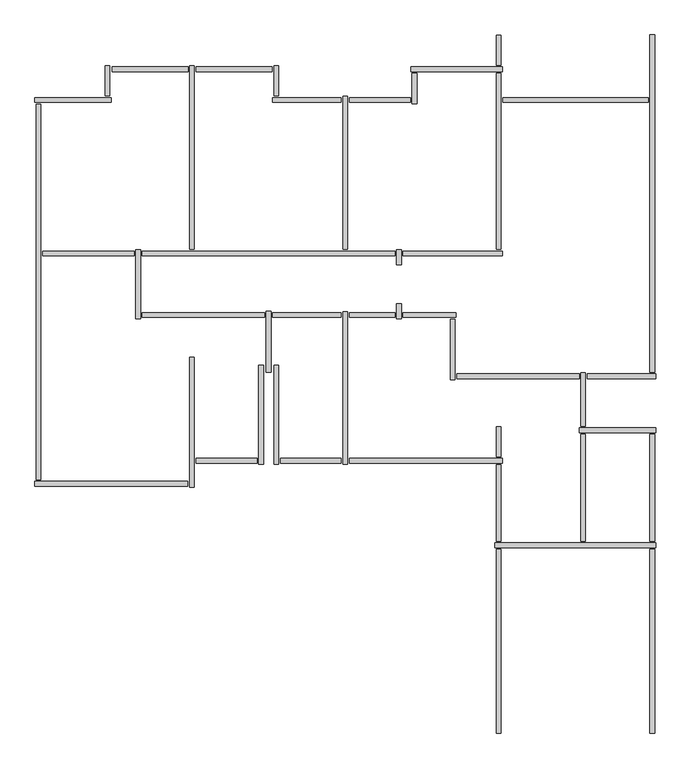
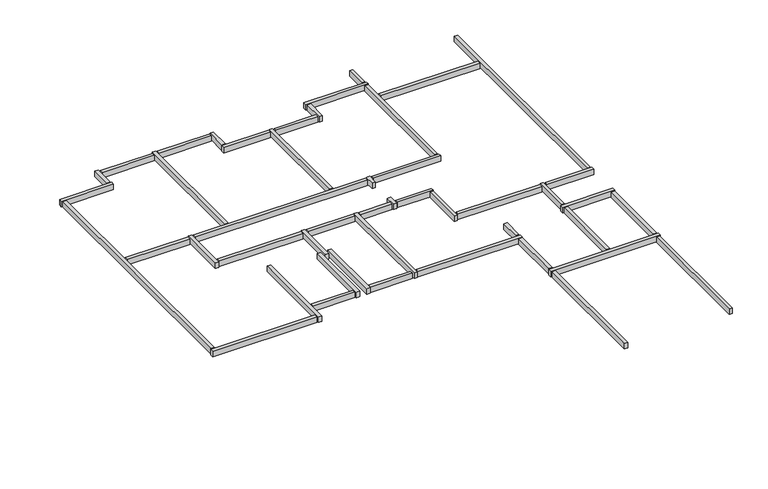
"""IFC4 building model written with IfcOpenShell, lengths in millimetres: beam geometry, Graute viga de respaldo19 : Graute viga de respaldo."""

from ifc_helpers import new_model, si_unit, frame, origin, place, context, project, spatial, polyline, outline, extrude, source, transform, mapped, element, save


def beam_b2c9fdfa(model_context):
    return source(origin(), model_context, "Body", "SweptSolid", [
        extrude(outline(polyline([(-70718.7587292, 62785.4278788), (-70624.7587292, 62785.4278788), (-70624.7587292, 59195.4278788), (-70718.7587292, 59195.4278788), (-70718.7587292, 62785.4278788)])), frame((0.0, 0.0, 14632.9999999), z_axis=(0.0, 0.0, 1.0), x_axis=(1.0, 0.0, 0.0)), (0.0, 0.0, 1.0), 167.0),
        extrude(outline(polyline([(-67718.7587292, 62785.4278788), (-67624.7587292, 62785.4278788), (-67624.7587292, 59195.4278788), (-67718.7587292, 59195.4278788), (-67718.7587292, 62785.4278788)])), frame((0.0, 0.0, 14632.9999999), z_axis=(0.0, 0.0, 1.0), x_axis=(1.0, 0.0, 0.0)), (0.0, 0.0, 1.0), 167.0),
        extrude(outline(polyline([(-75401.7587292, 64562.4278788), (-75401.7587292, 64468.4278788), (-76591.7587292, 64468.4278788), (-76591.7587292, 64562.4278788), (-75401.7587292, 64562.4278788)])), frame((0.0, 0.0, 14632.9999999), z_axis=(0.0, 0.0, 1.0), x_axis=(1.0, 0.0, 0.0)), (0.0, 0.0, 1.0), 167.0),
        extrude(outline(polyline([(-73751.7587292, 64562.4278788), (-73751.7587292, 64468.4278788), (-74941.7587292, 64468.4278788), (-74941.7587292, 64562.4278788), (-73751.7587292, 64562.4278788)])), frame((0.0, 0.0, 14632.9999999), z_axis=(0.0, 0.0, 1.0), x_axis=(1.0, 0.0, 0.0)), (0.0, 0.0, 1.0), 167.0),
        extrude(outline(polyline([(-77801.7587292, 68612.4278788), (-77801.7587292, 68518.4278788), (-79591.7587292, 68518.4278788), (-79591.7587292, 68612.4278788), (-77801.7587292, 68612.4278788)])), frame((0.0, 0.0, 14632.9999999), z_axis=(0.0, 0.0, 1.0), x_axis=(1.0, 0.0, 0.0)), (0.0, 0.0, 1.0), 167.0),
        extrude(outline(polyline([(-72401.7587292, 71612.4278788), (-72401.7587292, 71518.4278788), (-73591.7587292, 71518.4278788), (-73591.7587292, 71612.4278788), (-72401.7587292, 71612.4278788)])), frame((0.0, 0.0, 14632.9999999), z_axis=(0.0, 0.0, 1.0), x_axis=(1.0, 0.0, 0.0)), (0.0, 0.0, 1.0), 167.0),
        extrude(outline(polyline([(-72274.7587292, 71495.4278788), (-72368.7587292, 71495.4278788), (-72368.7587292, 72085.4278788), (-72274.7587292, 72085.4278788), (-72274.7587292, 71495.4278788)])), frame((0.0, 0.0, 14632.9999999), z_axis=(0.0, 0.0, 1.0), x_axis=(1.0, 0.0, 0.0)), (0.0, 0.0, 1.0), 167.0),
        extrude(outline(polyline([(-70601.7587292, 72212.4278788), (-70601.7587292, 72118.4278788), (-72391.7587292, 72118.4278788), (-72391.7587292, 72212.4278788), (-70601.7587292, 72212.4278788)])), frame((0.0, 0.0, 14632.9999999), z_axis=(0.0, 0.0, 1.0), x_axis=(1.0, 0.0, 0.0)), (0.0, 0.0, 1.0), 167.0),
        extrude(outline(polyline([(-72668.7587292, 68635.4278788), (-72574.7587292, 68635.4278788), (-72574.7587292, 68345.4278788), (-72668.7587292, 68345.4278788), (-72668.7587292, 68635.4278788)])), frame((0.0, 0.0, 14632.9999999), z_axis=(0.0, 0.0, 1.0), x_axis=(1.0, 0.0, 0.0)), (0.0, 0.0, 1.0), 167.0),
        extrude(outline(polyline([(-75251.7587292, 67412.4278788), (-75251.7587292, 67318.4278788), (-77641.7587292, 67318.4278788), (-77641.7587292, 67412.4278788), (-75251.7587292, 67412.4278788)])), frame((0.0, 0.0, 14632.9999999), z_axis=(0.0, 0.0, 1.0), x_axis=(1.0, 0.0, 0.0)), (0.0, 0.0, 1.0), 167.0),
        extrude(outline(polyline([(-73751.7587292, 67412.4278788), (-73751.7587292, 67318.4278788), (-75091.7587292, 67318.4278788), (-75091.7587292, 67412.4278788), (-73751.7587292, 67412.4278788)])), frame((0.0, 0.0, 14632.9999999), z_axis=(0.0, 0.0, 1.0), x_axis=(1.0, 0.0, 0.0)), (0.0, 0.0, 1.0), 167.0),
        extrude(outline(polyline([(-72701.7587292, 67412.4278788), (-72701.7587292, 67318.4278788), (-73591.7587292, 67318.4278788), (-73591.7587292, 67412.4278788), (-72701.7587292, 67412.4278788)])), frame((0.0, 0.0, 14632.9999999), z_axis=(0.0, 0.0, 1.0), x_axis=(1.0, 0.0, 0.0)), (0.0, 0.0, 1.0), 167.0),
        extrude(outline(polyline([(-72668.7587292, 67585.4278788), (-72574.7587292, 67585.4278788), (-72574.7587292, 67295.4278788), (-72668.7587292, 67295.4278788), (-72668.7587292, 67585.4278788)])), frame((0.0, 0.0, 14632.9999999), z_axis=(0.0, 0.0, 1.0), x_axis=(1.0, 0.0, 0.0)), (0.0, 0.0, 1.0), 167.0),
        extrude(outline(polyline([(-71511.7587292, 67412.4278788), (-71511.7587292, 67318.4278788), (-72541.7587292, 67318.4278788), (-72541.7587292, 67412.4278788), (-71511.7587292, 67412.4278788)])), frame((0.0, 0.0, 14632.9999999), z_axis=(0.0, 0.0, 1.0), x_axis=(1.0, 0.0, 0.0)), (0.0, 0.0, 1.0), 167.0),
        extrude(outline(polyline([(-71524.7587292, 66095.4278788), (-71618.7587292, 66095.4278788), (-71618.7587292, 67285.4278788), (-71524.7587292, 67285.4278788), (-71524.7587292, 66095.4278788)])), frame((0.0, 0.0, 14632.9999999), z_axis=(0.0, 0.0, 1.0), x_axis=(1.0, 0.0, 0.0)), (0.0, 0.0, 1.0), 167.0),
        extrude(outline(polyline([(-69091.7587292, 66212.4278788), (-69091.7587292, 66118.4278788), (-71491.7587292, 66118.4278788), (-71491.7587292, 66212.4278788), (-69091.7587292, 66212.4278788)])), frame((0.0, 0.0, 14632.9999999), z_axis=(0.0, 0.0, 1.0), x_axis=(1.0, 0.0, 0.0)), (0.0, 0.0, 1.0), 167.0),
        extrude(outline(polyline([(-73718.7587292, 67430.4278788), (-73624.7587292, 67430.4278788), (-73624.7587292, 64445.4278788), (-73718.7587292, 64445.4278788), (-73718.7587292, 67430.4278788)])), frame((0.0, 0.0, 14632.9999999), z_axis=(0.0, 0.0, 1.0), x_axis=(1.0, 0.0, 0.0)), (0.0, 0.0, 1.0), 167.0),
        extrude(outline(polyline([(-70601.7587292, 64562.4278788), (-70601.7587292, 64468.4278788), (-73591.7587292, 64468.4278788), (-73591.7587292, 64562.4278788), (-70601.7587292, 64562.4278788)])), frame((0.0, 0.0, 14632.9999999), z_axis=(0.0, 0.0, 1.0), x_axis=(1.0, 0.0, 0.0)), (0.0, 0.0, 1.0), 167.0),
        extrude(outline(polyline([(-70718.7587292, 65185.4278788), (-70624.7587292, 65185.4278788), (-70624.7587292, 64595.4278788), (-70718.7587292, 64595.4278788), (-70718.7587292, 65185.4278788)])), frame((0.0, 0.0, 14632.9999999), z_axis=(0.0, 0.0, 1.0), x_axis=(1.0, 0.0, 0.0)), (0.0, 0.0, 1.0), 167.0),
        extrude(outline(polyline([(-70624.7587292, 62945.4278788), (-70718.7587292, 62945.4278788), (-70718.7587292, 64435.4278788), (-70624.7587292, 64435.4278788), (-70624.7587292, 62945.4278788)])), frame((0.0, 0.0, 14632.9999999), z_axis=(0.0, 0.0, 1.0), x_axis=(1.0, 0.0, 0.0)), (0.0, 0.0, 1.0), 167.0),
        extrude(outline(polyline([(-67624.7587292, 62945.4278788), (-67718.7587292, 62945.4278788), (-67718.7587292, 65035.4278788), (-67624.7587292, 65035.4278788), (-67624.7587292, 62945.4278788)])), frame((0.0, 0.0, 14632.9999999), z_axis=(0.0, 0.0, 1.0), x_axis=(1.0, 0.0, 0.0)), (0.0, 0.0, 1.0), 167.0),
        extrude(outline(polyline([(-68974.7587292, 62945.4278788), (-69068.7587292, 62945.4278788), (-69068.7587292, 65035.4278788), (-68974.7587292, 65035.4278788), (-68974.7587292, 62945.4278788)])), frame((0.0, 0.0, 14632.9999999), z_axis=(0.0, 0.0, 1.0), x_axis=(1.0, 0.0, 0.0)), (0.0, 0.0, 1.0), 167.0),
        extrude(outline(polyline([(-69068.7587292, 66235.4278788), (-68974.7587292, 66235.4278788), (-68974.7587292, 65195.4278788), (-69068.7587292, 65195.4278788), (-69068.7587292, 66235.4278788)])), frame((0.0, 0.0, 14632.9999999), z_axis=(0.0, 0.0, 1.0), x_axis=(1.0, 0.0, 0.0)), (0.0, 0.0, 1.0), 167.0),
        extrude(outline(polyline([(-67751.7587292, 71612.4278788), (-67751.7587292, 71518.4278788), (-70591.7587292, 71518.4278788), (-70591.7587292, 71612.4278788), (-67751.7587292, 71612.4278788)])), frame((0.0, 0.0, 14632.9999999), z_axis=(0.0, 0.0, 1.0), x_axis=(1.0, 0.0, 0.0)), (0.0, 0.0, 1.0), 167.0),
        extrude(outline(polyline([(-70624.7587292, 68645.4278788), (-70718.7587292, 68645.4278788), (-70718.7587292, 72085.4278788), (-70624.7587292, 72085.4278788), (-70624.7587292, 68645.4278788)])), frame((0.0, 0.0, 14632.9999999), z_axis=(0.0, 0.0, 1.0), x_axis=(1.0, 0.0, 0.0)), (0.0, 0.0, 1.0), 167.0),
        extrude(outline(polyline([(-70601.7587292, 68612.4278788), (-70601.7587292, 68518.4278788), (-72541.7587292, 68518.4278788), (-72541.7587292, 68612.4278788), (-70601.7587292, 68612.4278788)])), frame((0.0, 0.0, 14632.9999999), z_axis=(0.0, 0.0, 1.0), x_axis=(1.0, 0.0, 0.0)), (0.0, 0.0, 1.0), 167.0),
        extrude(outline(polyline([(-72701.7587292, 68612.4278788), (-72701.7587292, 68518.4278788), (-77641.7587292, 68518.4278788), (-77641.7587292, 68612.4278788), (-72701.7587292, 68612.4278788)])), frame((0.0, 0.0, 14632.9999999), z_axis=(0.0, 0.0, 1.0), x_axis=(1.0, 0.0, 0.0)), (0.0, 0.0, 1.0), 167.0),
        extrude(outline(polyline([(-73718.7587292, 71635.4278788), (-73624.7587292, 71635.4278788), (-73624.7587292, 68645.4278788), (-73718.7587292, 68645.4278788), (-73718.7587292, 71635.4278788)])), frame((0.0, 0.0, 14632.9999999), z_axis=(0.0, 0.0, 1.0), x_axis=(1.0, 0.0, 0.0)), (0.0, 0.0, 1.0), 167.0),
        extrude(outline(polyline([(-75091.7587292, 71518.4278788), (-75091.7587292, 71612.4278788), (-73751.7587292, 71612.4278788), (-73751.7587292, 71518.4278788), (-75091.7587292, 71518.4278788)])), frame((0.0, 0.0, 14632.9999999), z_axis=(0.0, 0.0, 1.0), x_axis=(1.0, 0.0, 0.0)), (0.0, 0.0, 1.0), 167.0),
        extrude(outline(polyline([(-75068.7587292, 72235.4278788), (-74974.7587292, 72235.4278788), (-74974.7587292, 71645.4278788), (-75068.7587292, 71645.4278788), (-75068.7587292, 72235.4278788)])), frame((0.0, 0.0, 14632.9999999), z_axis=(0.0, 0.0, 1.0), x_axis=(1.0, 0.0, 0.0)), (0.0, 0.0, 1.0), 167.0),
        extrude(outline(polyline([(-75101.7587292, 72212.4278788), (-75101.7587292, 72118.4278788), (-76591.7587292, 72118.4278788), (-76591.7587292, 72212.4278788), (-75101.7587292, 72212.4278788)])), frame((0.0, 0.0, 14632.9999999), z_axis=(0.0, 0.0, 1.0), x_axis=(1.0, 0.0, 0.0)), (0.0, 0.0, 1.0), 167.0),
        extrude(outline(polyline([(-78230.736554, 72117.4278788), (-78230.736554, 72212.4278788), (-76741.7587292, 72212.4278788), (-76741.7587292, 72117.4278788), (-78230.736554, 72117.4278788)])), frame((0.0, 0.0, 14617.1856208), z_axis=(0.0, 0.0, 1.0), x_axis=(1.0, 0.0, 0.0)), (0.0, 0.0, 1.0), 165.0),
        extrude(outline(polyline([(-79624.7587292, 64145.4278788), (-79718.7587292, 64145.4278788), (-79718.7587292, 71485.4278788), (-79624.7587292, 71485.4278788), (-79624.7587292, 64145.4278788)])), frame((0.0, 0.0, 14632.9999999), z_axis=(0.0, 0.0, 1.0), x_axis=(1.0, 0.0, 0.0)), (0.0, 0.0, 1.0), 167.0),
        extrude(outline(polyline([(-77674.7587292, 67295.4278788), (-77768.7587292, 67295.4278788), (-77768.7587292, 68640.7810915), (-77674.7587292, 68640.7810915), (-77674.7587292, 67295.4278788)])), frame((0.0, 0.0, 14632.9999999), z_axis=(0.0, 0.0, 1.0), x_axis=(1.0, 0.0, 0.0)), (0.0, 0.0, 1.0), 167.0),
        extrude(outline(polyline([(-75124.7587292, 66245.4278788), (-75218.7587292, 66245.4278788), (-75218.7587292, 67435.4278788), (-75124.7587292, 67435.4278788), (-75124.7587292, 66245.4278788)])), frame((0.0, 0.0, 14632.9999999), z_axis=(0.0, 0.0, 1.0), x_axis=(1.0, 0.0, 0.0)), (0.0, 0.0, 1.0), 167.0),
        extrude(outline(polyline([(-75274.7587292, 64445.4278788), (-75368.7587292, 64445.4278788), (-75368.7587292, 66385.4278788), (-75274.7587292, 66385.4278788), (-75274.7587292, 64445.4278788)])), frame((0.0, 0.0, 14632.9999999), z_axis=(0.0, 0.0, 1.0), x_axis=(1.0, 0.0, 0.0)), (0.0, 0.0, 1.0), 167.0),
        extrude(outline(polyline([(-74974.7587292, 64445.4278788), (-75068.7587292, 64445.4278788), (-75068.7587292, 66385.4278788), (-74974.7587292, 66385.4278788), (-74974.7587292, 64445.4278788)])), frame((0.0, 0.0, 14632.9999999), z_axis=(0.0, 0.0, 1.0), x_axis=(1.0, 0.0, 0.0)), (0.0, 0.0, 1.0), 167.0),
        extrude(outline(polyline([(-76624.7587292, 63995.4278788), (-76718.7587292, 63995.4278788), (-76718.7587292, 66535.4278788), (-76624.7587292, 66535.4278788), (-76624.7587292, 63995.4278788)])), frame((0.0, 0.0, 14632.9999999), z_axis=(0.0, 0.0, 1.0), x_axis=(1.0, 0.0, 0.0)), (0.0, 0.0, 1.0), 167.0),
        extrude(outline(polyline([(-79741.7587292, 64018.4278788), (-79741.7587292, 64112.4278788), (-76751.7587292, 64112.4278788), (-76751.7587292, 64018.4278788), (-79741.7587292, 64018.4278788)])), frame((0.0, 0.0, 14632.9999999), z_axis=(0.0, 0.0, 1.0), x_axis=(1.0, 0.0, 0.0)), (0.0, 0.0, 1.0), 167.0),
        extrude(outline(polyline([(-78368.7587292, 72235.4278788), (-78274.7587292, 72235.4278788), (-78274.7587292, 71645.4278788), (-78368.7587292, 71645.4278788), (-78368.7587292, 72235.4278788)])), frame((0.0, 0.0, 14632.9999999), z_axis=(0.0, 0.0, 1.0), x_axis=(1.0, 0.0, 0.0)), (0.0, 0.0, 1.0), 167.0),
        extrude(outline(polyline([(-78251.7587292, 71612.4278788), (-78251.7587292, 71518.4278788), (-79741.7587292, 71518.4278788), (-79741.7587292, 71612.4278788), (-78251.7587292, 71612.4278788)])), frame((0.0, 0.0, 14632.9999999), z_axis=(0.0, 0.0, 1.0), x_axis=(1.0, 0.0, 0.0)), (0.0, 0.0, 1.0), 167.0),
        extrude(outline(polyline([(-76718.7587292, 72235.4278788), (-76624.7587292, 72235.4278788), (-76624.7587292, 68645.4278788), (-76718.7587292, 68645.4278788), (-76718.7587292, 72235.4278788)])), frame((0.0, 0.0, 14632.9999999), z_axis=(0.0, 0.0, 1.0), x_axis=(1.0, 0.0, 0.0)), (0.0, 0.0, 1.0), 167.0),
        extrude(outline(polyline([(-70718.7587292, 72835.4278788), (-70624.7587292, 72835.4278788), (-70624.7587292, 72245.4278788), (-70718.7587292, 72245.4278788), (-70718.7587292, 72835.4278788)])), frame((0.0, 0.0, 14632.9999999), z_axis=(0.0, 0.0, 1.0), x_axis=(1.0, 0.0, 0.0)), (0.0, 0.0, 1.0), 167.0),
        extrude(outline(polyline([(-67601.7587292, 65162.4278788), (-67601.7587292, 65068.4278788), (-69091.7587292, 65068.4278788), (-69091.7587292, 65162.4278788), (-67601.7587292, 65162.4278788)])), frame((0.0, 0.0, 14632.9999999), z_axis=(0.0, 0.0, 1.0), x_axis=(1.0, 0.0, 0.0)), (0.0, 0.0, 1.0), 167.0),
        extrude(outline(polyline([(-67601.7587292, 62912.4278788), (-67601.7587292, 62818.4278788), (-70741.7587292, 62818.4278788), (-70741.7587292, 62912.4278788), (-67601.7587292, 62912.4278788)])), frame((0.0, 0.0, 14632.9999999), z_axis=(0.0, 0.0, 1.0), x_axis=(1.0, 0.0, 0.0)), (0.0, 0.0, 1.0), 167.0),
        extrude(outline(polyline([(-67601.7587292, 66212.4278788), (-67601.7587292, 66118.4278788), (-68941.7587292, 66118.4278788), (-68941.7587292, 66212.4278788), (-67601.7587292, 66212.4278788)])), frame((0.0, 0.0, 14632.9999999), z_axis=(0.0, 0.0, 1.0), x_axis=(1.0, 0.0, 0.0)), (0.0, 0.0, 1.0), 167.0),
        extrude(outline(polyline([(-67718.7587292, 72837.9577736), (-67624.7587292, 72837.9577736), (-67624.7587292, 66245.4278788), (-67718.7587292, 66245.4278788), (-67718.7587292, 72837.9577736)])), frame((0.0, 0.0, 14632.9999999), z_axis=(0.0, 0.0, 1.0), x_axis=(1.0, 0.0, 0.0)), (0.0, 0.0, 1.0), 167.0),
    ])


if __name__ == "__main__":
    model = new_model("IFC4")
    model_context = context("Model", 3, world=origin())
    ifc_project = project(units=[si_unit("LENGTHUNIT", "METRE", prefix="MILLI")], contexts=[model_context])
    site = spatial("IfcSite", under=ifc_project)
    building = spatial("IfcBuilding", under=site)
    placement = place(None, origin())
    beam_shape = beam_b2c9fdfa(model_context)
    element("IfcBeam", 1, ObjectType="Graute viga de respaldo19 : Graute viga de respaldo", at=placement, inside=building, context=model_context, shape_type="MappedRepresentation", body=[
        mapped(beam_shape, transform((0.0, 0.0, 0.0), x_axis=(1.0, 0.0, 0.0), y_axis=(0.0, 1.0, 0.0), z_axis=(0.0, 0.0, 1.0))),
    ])
    save(model, "model.ifc")

# Revit data of these elements
# Element 1 (IfcBeam, "Graute viga de respaldo19 : Graute viga de respaldo")
#   Materials on its faces: "Concreto, Faixa de areia/cimento"
# Materials
#   "Concreto, Faixa de areia/cimento": class "Concreto", colour RGB 127 127 127, transparency 0, Description = "Revestimento de laje de concreto", Cost = 0
